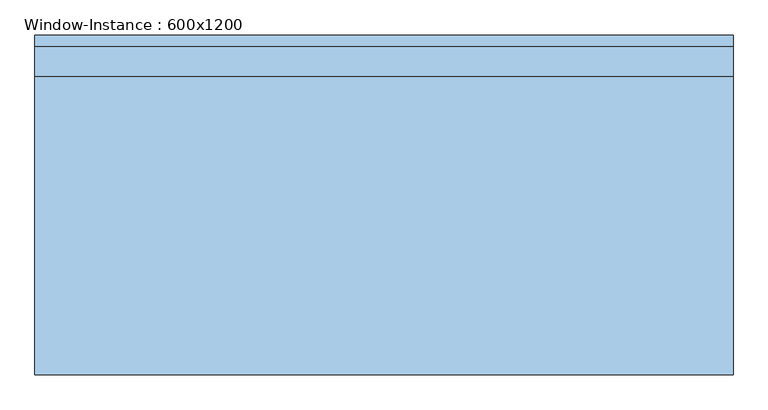
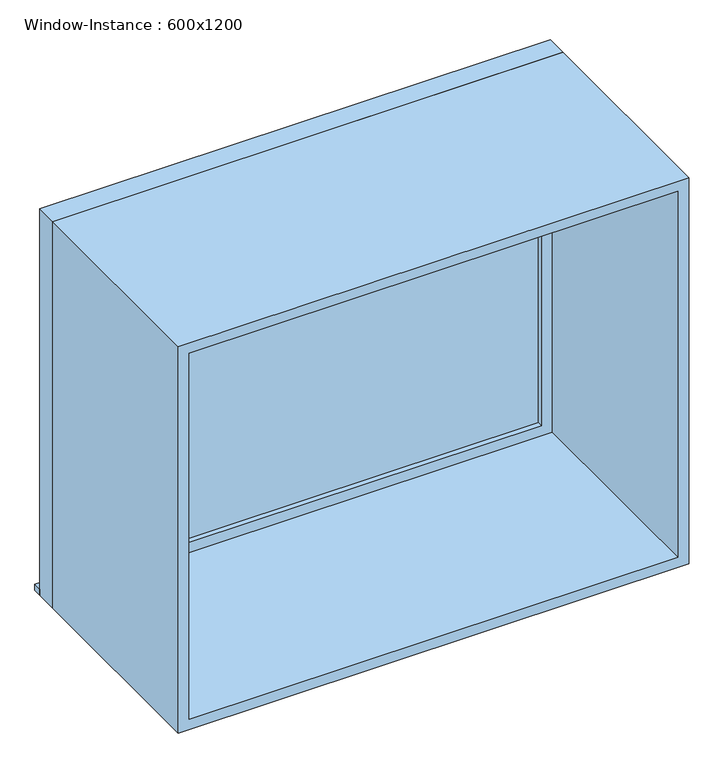
"""IFC4 building model written with IfcOpenShell, lengths in millimetres: window geometry, Window-Instance : 600x1200."""

from ifc_helpers import new_model, si_unit, frame, origin, place, context, project, spatial, polyline, outline, extrude, source, transform, mapped, element, save


def window_instance_600x1200_532ba9b3(model_context):
    return source(origin(), model_context, "Body", "SweptSolid", [
        extrude(outline(polyline([(-788.1, 377.9), (711.9, 377.9), (711.9, 352.5), (-788.1, 352.5), (-788.1, 377.9)])), frame((0.0, 0.0, 900.0), z_axis=(0.0, 0.0, 1.0), x_axis=(1.0, 0.0, 0.0)), (0.0, 0.0, 1.0), 19.05),
        extrude(outline(polyline([(648.4, 303.925), (-724.6, 303.925), (-724.6, 316.625), (648.4, 316.625), (648.4, 303.925)])), frame((0.0, 0.0, 963.5), z_axis=(0.0, 0.0, 1.0), x_axis=(1.0, 0.0, 0.0)), (0.0, 0.0, 1.0), 1073.0),
        extrude(outline(polyline([(2080.95, -769.05), (919.05, -769.05), (919.05, 692.85), (2080.95, 692.85), (2080.95, -769.05)]), holes=[polyline([(2036.5, -724.6), (2036.5, 648.4), (963.5, 648.4), (963.5, -724.6), (2036.5, -724.6)])]), frame((0.0, 288.05, 0.0), z_axis=(0.0, 1.0, 0.0), x_axis=(0.0, 0.0, 1.0)), (0.0, 0.0, 1.0), 44.45),
        extrude(outline(polyline([(2100.0, -788.1), (900.0, -788.1), (900.0, 711.9), (2100.0, 711.9), (2100.0, -788.1)]), holes=[polyline([(2068.25, -756.35), (2068.25, 680.15), (931.75, 680.15), (931.75, -756.35), (2068.25, -756.35)])]), frame((0.0, -352.5, 0.0), z_axis=(0.0, 1.0, 0.0), x_axis=(0.0, 0.0, 1.0)), (0.0, 0.0, 1.0), 640.55),
        extrude(outline(polyline([(2100.0, 711.9), (2100.0, -788.1), (900.0, -788.1), (900.0, 711.9), (2100.0, 711.9)]), holes=[polyline([(2080.95, 692.85), (919.05, 692.85), (919.05, -769.05), (2080.95, -769.05), (2080.95, 692.85)])]), frame((0.0, 288.05, 0.0), z_axis=(0.0, 1.0, 0.0), x_axis=(0.0, 0.0, 1.0)), (0.0, 0.0, 1.0), 64.45),
    ])


if __name__ == "__main__":
    model = new_model("IFC4")
    model_context = context("Model", 3, world=origin())
    ifc_project = project(units=[si_unit("LENGTHUNIT", "METRE", prefix="MILLI")], contexts=[model_context])
    site = spatial("IfcSite", under=ifc_project)
    building = spatial("IfcBuilding", under=site)
    placement = place(None, origin())
    window_instance_600x1200_shape = window_instance_600x1200_532ba9b3(model_context)
    element("IfcWindow", 1, ObjectType="Window-Instance : 600x1200", at=placement, inside=building, context=model_context, shape_type="MappedRepresentation", body=[
        mapped(window_instance_600x1200_shape, transform((0.0, 0.0, 0.0), x_axis=(1.0, 0.0, 0.0), y_axis=(0.0, 1.0, 0.0), z_axis=(0.0, 0.0, 1.0))),
    ])
    save(model, "model.ifc")

# Revit data of these elements
# Type "Window-Instance : 600x1200"
#   Type Mark = "7"
#   Construction Type Id = "GSP4R"
#   Assembly Code = "B2020100"
#   Analytic Construction = "1/8 in Pilkington single glazing"
#   Visual Light Transmittance = 0.9
#   Thermal Resistance (R) = 0.149095 (m²·K)/W
#   Solar Heat Gain Coefficient = 0.86
#   Heat Transfer Coefficient (U) = 6.70716 W/(m²·K)
#   Height [instance default] = 1200 mm
#   Default Sill Height = 900 mm
#   Width [instance default] = 600 mm
#   Window Inset = 20 mm
#   Glass Pane Material = WW-EC-GL-Storefront
#   Sash Material = WW-EC-RGB-White
#   Wall Closure = (empty or 0)
# Element 1 (IfcWindow, "Window-Instance : 600x1200")
#   Width = 1500 mm
#   Materials on its faces: "WW-EC-RGB-White", "WW-EC-GL-Storefront"
# Materials
#   "WW-EC-GL-Storefront": class "Glass", colour RGB 236 240 239, transparency 0.85, Description = "Storefront Glass", Cost = 0
#   "WW-EC-RGB-White": class "Generic", colour RGB 255 255 255, transparency 0, Comments = "If region requests off-white, swith asset color to RGB 231-228-220", Description = "Generic Color", Cost = 0
